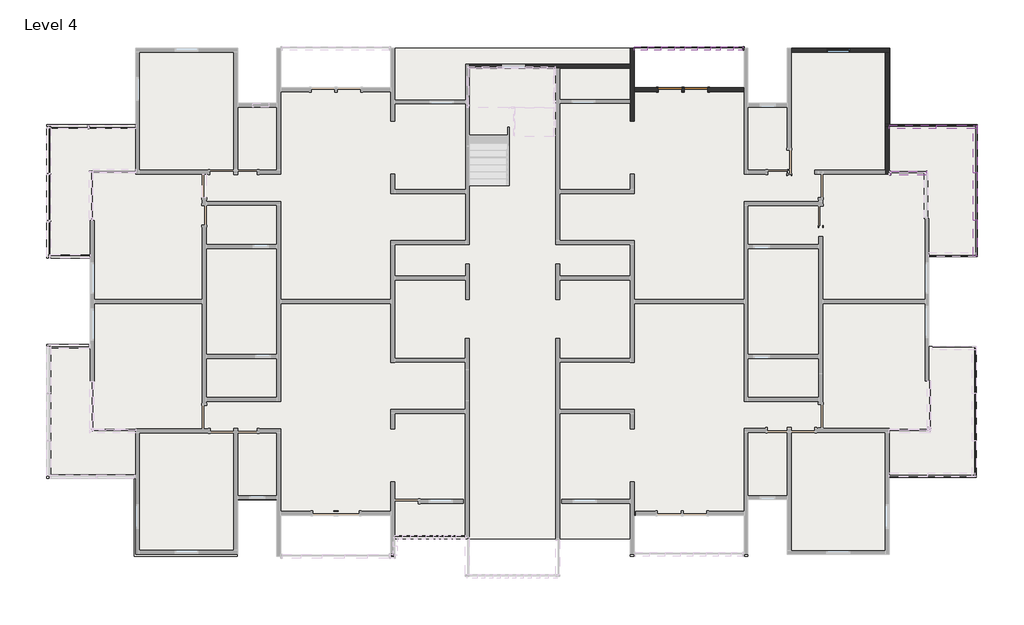
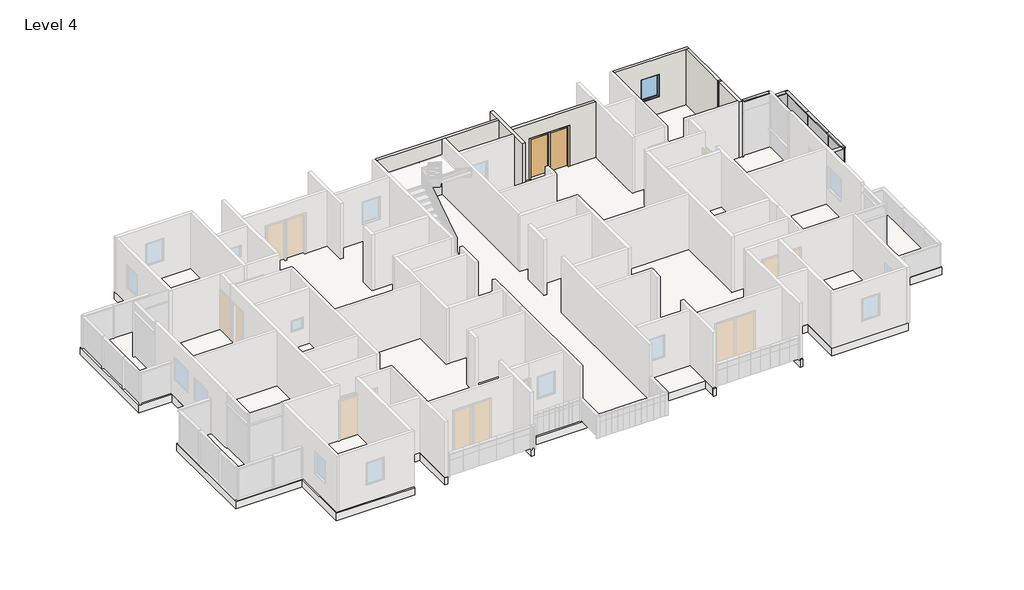
# One storey, part 5 of 7: 16 members, 15 plates, 7 walls, 2 doors, 1 slab, 1 window.
"""IFC4 building model written with IfcOpenShell, lengths in millimetres."""

import ifcopenshell
import ifcopenshell.guid

model = None  # the IFC model being written
_history = None  # IfcOwnerHistory: only IFC2X3 demands one
_inside = {}  # id of a spatial element -> (the spatial element, [elements in it])
_under = {}  # id of a project, library or spatial element -> (it, [spatial elements below it])
_declared = {}  # id of a project -> (the project, [libraries it declares])
_typed = {}  # id of a type object -> (the type object, [elements of that type])
_made_of = {}  # id of a material, layer set ... -> (it, [elements and type objects made of it])


def new_model(schema):
    """Start an empty IFC model of exactly this schema.

    Asked for "IFC4X3", IfcOpenShell would pick the latest addendum, in which some entities
    have other attributes; the version numbers below select the first issue.
    IFC2X3 requires an IfcOwnerHistory on every rooted entity: one is made here for all.
    """
    global model, _history
    if schema == "IFC4X3":
        model = ifcopenshell.file(schema_version=(4, 3, 0, 0))
    else:
        model = ifcopenshell.file(schema=schema)
    _inside.clear()
    _under.clear()
    _declared.clear()
    _typed.clear()
    _made_of.clear()
    _history = None
    if model.schema == "IFC2X3":
        org = make("IfcOrganization", Name="unknown")
        user = make(
            "IfcPersonAndOrganization",
            ThePerson=make("IfcPerson", FamilyName="unknown"),
            TheOrganization=org,
        )
        app = make(
            "IfcApplication",
            ApplicationDeveloper=org,
            Version="unknown",
            ApplicationFullName="unknown",
            ApplicationIdentifier="unknown",
        )
        _history = make(
            "IfcOwnerHistory",
            OwningUser=user,
            OwningApplication=app,
            ChangeAction="ADDED",
            CreationDate=0,
        )
    return model


def make(cls, **values):
    """One entity of the class cls with the attributes given. An attribute that is None is left unset."""
    return model.create_entity(
        cls, **{name: value for name, value in values.items() if value is not None}
    )


def rooted(cls, **values):
    """An entity with a GlobalId (a new one), such as an element, a storey or a relation."""
    return make(cls, GlobalId=ifcopenshell.guid.new(), OwnerHistory=_history, **values)


def si_unit(unit_type, name, prefix=None):
    """IfcSIUnit, for example si_unit("LENGTHUNIT", "METRE", prefix="MILLI")."""
    return make("IfcSIUnit", UnitType=unit_type, Prefix=prefix, Name=name)


def assignment(units):
    """IfcUnitAssignment: the units of a project."""
    return None if units is None else make("IfcUnitAssignment", Units=units)


def point(xyz):
    """IfcCartesianPoint."""
    return None if xyz is None else make("IfcCartesianPoint", Coordinates=xyz)


def direction(xyz):
    """IfcDirection."""
    return None if xyz is None else make("IfcDirection", DirectionRatios=xyz)


def frame(location, z_axis=None, x_axis=None):
    """IfcAxis2Placement3D, a coordinate frame: its origin and axes. An axis left out is left unset."""
    return make(
        "IfcAxis2Placement3D",
        Location=point(location),
        Axis=direction(z_axis),
        RefDirection=direction(x_axis),
    )


def origin():
    """The frame at (0, 0, 0) with its axes left unset."""
    return frame((0.0, 0.0, 0.0))


def origin_with_axes():
    """The frame at (0, 0, 0) with the z axis (0, 0, 1) and the x axis (1, 0, 0) written out."""
    return frame((0.0, 0.0, 0.0), z_axis=(0.0, 0.0, 1.0), x_axis=(1.0, 0.0, 0.0))


def place(relative_to, where):
    """IfcLocalPlacement: puts the frame where relative to a parent placement (None: the world)."""
    return make(
        "IfcLocalPlacement", PlacementRelTo=relative_to, RelativePlacement=where
    )


def context(
    kind, dimensions, precision=None, world=None, true_north=None, identifier=None
):
    """IfcGeometricRepresentationContext, for example the 3D "Model" context."""
    return make(
        "IfcGeometricRepresentationContext",
        ContextIdentifier=identifier,
        ContextType=kind,
        CoordinateSpaceDimension=dimensions,
        Precision=precision,
        WorldCoordinateSystem=world,
        TrueNorth=true_north,
    )


def project(units=None, contexts=None):
    """IfcProject with its units and contexts."""
    return rooted(
        "IfcProject",
        Name="project",
        RepresentationContexts=contexts,
        UnitsInContext=assignment(units),
    )


def spatial(cls, under=None, at=None, **own):
    """A site, building, storey or space (cls), placed at a placement, below another one or the project."""
    s = rooted(cls, ObjectPlacement=at, **own)
    if under is not None:
        _under.setdefault(under.id(), (under, []))[1].append(s)
    return s


def polyline(points):
    """IfcPolyline through the points."""
    return make("IfcPolyline", Points=[point(p) for p in points])


def outline(outer, holes=None, kind="AREA"):
    """IfcArbitraryClosedProfileDef: a profile drawn as a closed curve; with holes, ...WithVoids."""
    if holes is None:
        return make("IfcArbitraryClosedProfileDef", ProfileType=kind, OuterCurve=outer)
    return make(
        "IfcArbitraryProfileDefWithVoids",
        ProfileType=kind,
        OuterCurve=outer,
        InnerCurves=holes,
    )


def extrude(swept, where, along, depth):
    """IfcExtrudedAreaSolid: the profile swept, set in the frame where, extruded along a direction by depth."""
    return make(
        "IfcExtrudedAreaSolid",
        SweptArea=swept,
        Position=where,
        ExtrudedDirection=direction(along),
        Depth=depth,
    )


def faces_of(points, faces, orient=None, outer=None):
    """IfcFace entities. A face is a list of loops; a loop is a list of indices into points, from 0.

    orient and outer hold one flag for each loop. By default every Orientation is true, the
    first loop of a face is its IfcFaceOuterBound and the others are IfcFaceBound.
    """
    made = []
    for i, loops in enumerate(faces):
        bounds = []
        for j, loop in enumerate(loops):
            is_outer = j == 0 if outer is None else outer[i][j]
            bounds.append(
                make(
                    "IfcFaceOuterBound" if is_outer else "IfcFaceBound",
                    Bound=make("IfcPolyLoop", Polygon=[points[k] for k in loop]),
                    Orientation=True if orient is None else orient[i][j],
                )
            )
        made.append(make("IfcFace", Bounds=bounds))
    return made


def faceted_brep(points, faces, orient=None, outer=None, voids=None):
    """IfcFacetedBrep: a solid bounded by flat faces; with voids (closed shells), ...WithVoids."""
    shared = [point(p) for p in points]
    hull = make("IfcClosedShell", CfsFaces=faces_of(shared, faces, orient, outer))
    if voids is None:
        return make("IfcFacetedBrep", Outer=hull)
    return make(
        "IfcFacetedBrepWithVoids",
        Outer=hull,
        Voids=[
            make(cls, CfsFaces=faces_of(shared, fs, o, b)) for cls, fs, o, b in voids
        ],
    )


def shape(context_of_items, identifier, shape_type, items):
    """IfcShapeRepresentation: the items that make up one representation, for example the "Body"."""
    return make(
        "IfcShapeRepresentation",
        ContextOfItems=context_of_items,
        RepresentationIdentifier=identifier,
        RepresentationType=shape_type,
        Items=items,
    )


def source(mapping_origin, context_of_items, identifier, shape_type, items):
    """IfcRepresentationMap: a shape defined once, which mapped items show again and again."""
    return make(
        "IfcRepresentationMap",
        MappingOrigin=mapping_origin,
        MappedRepresentation=shape(context_of_items, identifier, shape_type, items),
    )


def transform(
    local_origin,
    x_axis=None,
    y_axis=None,
    z_axis=None,
    scale=None,
    scale2=None,
    scale3=None,
    uniform=True,
):
    """IfcCartesianTransformationOperator3D, or its non-uniform kind. x_axis, y_axis, z_axis: its Axis1, 2, 3."""
    if uniform:
        return make(
            "IfcCartesianTransformationOperator3D",
            Axis1=direction(x_axis),
            Axis2=direction(y_axis),
            LocalOrigin=point(local_origin),
            Scale=scale,
            Axis3=direction(z_axis),
        )
    return make(
        "IfcCartesianTransformationOperator3DnonUniform",
        Axis1=direction(x_axis),
        Axis2=direction(y_axis),
        LocalOrigin=point(local_origin),
        Scale=scale,
        Axis3=direction(z_axis),
        Scale2=scale2,
        Scale3=scale3,
    )


def mapped(mapping_source, mapping_target):
    """IfcMappedItem: shows the shape of a source again, moved by a transform."""
    return make(
        "IfcMappedItem", MappingSource=mapping_source, MappingTarget=mapping_target
    )


def made_of(thing, what):
    """Note that an element or type object is made of a material, layer set ...; save() writes the relation."""
    if what is not None:
        _made_of.setdefault(what.id(), (what, []))[1].append(thing)
    return thing


def element(
    cls,
    number,
    at=None,
    inside=None,
    cuts=None,
    type_object=None,
    material=None,
    context=None,
    identifier="Body",
    shape_type=None,
    held_by="IfcProductDefinitionShape",
    body=None,
    shapes=None,
    **own,
):
    """One element of the class cls, such as IfcWall. Its Tag is "e" and its number.

    at: its placement. inside: the storey or other place that contains it. cuts: it is an
    opening in that element (IfcRelVoidsElement). A single representation is given by context,
    identifier, shape_type and body (its items); several are given by shapes. held_by: the class
    of the entity that holds the representations. save() writes the other relations.
    """
    e = rooted(cls, Tag="e%d" % number, ObjectPlacement=at, **own)
    if body is not None:
        shapes = [shape(context, identifier, shape_type, body)]
    if shapes is not None:
        e.Representation = make(held_by, Representations=shapes)
    if inside is not None:
        _inside.setdefault(inside.id(), (inside, []))[1].append(e)
    if cuts is not None:
        rooted(
            "IfcRelVoidsElement", RelatingBuildingElement=cuts, RelatedOpeningElement=e
        )
    if type_object is not None:
        _typed.setdefault(type_object.id(), (type_object, []))[1].append(e)
    return made_of(e, material)


def aggregate(whole, parts):
    """IfcRelAggregates: a whole, such as a stair, and the parts it consists of."""
    return rooted("IfcRelAggregates", RelatingObject=whole, RelatedObjects=parts)


def save(model, path):
    """Write the relations noted so far, then the file.

    IfcRelAggregates (storeys below a building ...), IfcRelContainedInSpatialStructure (elements
    in a storey), IfcRelDefinesByType, IfcRelAssociatesMaterial and IfcRelDeclares: one each for
    every whole, place, type object, material and project.
    """
    for whole, parts in _under.values():
        aggregate(whole, parts)
    for where, things in _inside.values():
        rooted(
            "IfcRelContainedInSpatialStructure",
            RelatedElements=things,
            RelatingStructure=where,
        )
    for kind, things in _typed.values():
        rooted("IfcRelDefinesByType", RelatedObjects=things, RelatingType=kind)
    for what, things in _made_of.values():
        rooted("IfcRelAssociatesMaterial", RelatedObjects=things, RelatingMaterial=what)
    for by, libraries in _declared.values():
        rooted("IfcRelDeclares", RelatingContext=by, RelatedDefinitions=libraries)
    model.write(path)


def m_single_flush_0915_x_2134mm_138fd904(model_context):
    return source(origin(), model_context, "Body", "SweptSolid", [
        extrude(outline(polyline([(2210.0, -533.5), (0.0, -533.5), (0.0, -457.5), (2134.0, -457.5), (2134.0, 457.5), (0.0, 457.5), (0.0, 533.5), (2210.0, 533.5), (2210.0, -533.5)])), frame((0.0, 75.0, 0.0), z_axis=(0.0, 1.0, 0.0), x_axis=(0.0, 0.0, 1.0)), (0.0, 0.0, 1.0), 25.0),
        extrude(outline(polyline([(2210.0, 533.5), (2210.0, -533.5), (0.0, -533.5), (0.0, -457.5), (2134.0, -457.5), (2134.0, 457.5), (0.0, 457.5), (0.0, 533.5), (2210.0, 533.5)])), frame((0.0, -100.0, 0.0), z_axis=(0.0, 1.0, 0.0), x_axis=(0.0, 0.0, 1.0)), (0.0, 0.0, 1.0), 25.0),
        extrude(outline(polyline([(457.5, 24.0), (-457.5, 24.0), (-457.5, 75.0), (457.5, 75.0), (457.5, 24.0)])), origin_with_axes(), (0.0, 0.0, 1.0), 2134.0),
    ])


def rectangular_mullion_50mm_x_150mm_42770ee2(model_context):
    return source(origin(), model_context, "Body", "SweptSolid", [
        extrude(outline(polyline([(0.0, 75.0), (0.0, -75.0), (-50.0, -75.0), (-50.0, 75.0), (0.0, 75.0)])), frame((0.0, 0.0, -1830.0000003), z_axis=(0.0, 0.0, 1.0), x_axis=(1.0, 0.0, 0.0)), (0.0, 0.0, 1.0), 1830.0000003),
    ])


def rectangular_mullion_50mm_x_150mm_aaee7d48(model_context):
    return source(origin(), model_context, "Body", "SweptSolid", [
        extrude(outline(polyline([(0.0, 75.0), (0.0, -75.0), (-50.0, -75.0), (-50.0, 75.0), (0.0, 75.0)])), frame((0.0, 0.0, -1830.0), z_axis=(0.0, 0.0, 1.0), x_axis=(1.0, 0.0, 0.0)), (0.0, 0.0, 1.0), 1830.0),
    ])


def rectangular_mullion_50mm_x_150mm_efa02866(model_context):
    return source(origin(), model_context, "Body", "SweptSolid", [
        extrude(outline(polyline([(0.0, 75.0), (0.0, -75.0), (-50.0, -75.0), (-50.0, 75.0), (0.0, 75.0)])), frame((0.0, 0.0, -1399.9999997), z_axis=(0.0, 0.0, 1.0), x_axis=(1.0, 0.0, 0.0)), (0.0, 0.0, 1.0), 1399.9999997),
    ])


def rectangular_mullion_50mm_x_150mm_d9f1e9e9(model_context):
    return source(origin(), model_context, "Body", "SweptSolid", [
        extrude(outline(polyline([(0.0, 75.0), (0.0, -75.0), (-50.0, -75.0), (-50.0, 75.0), (0.0, 75.0)])), frame((0.0, 0.0, -1565.8160321), z_axis=(0.0, 0.0, 1.0), x_axis=(1.0, 0.0, 0.0)), (0.0, 0.0, 1.0), 1565.8160321),
    ])


def rectangular_mullion_50mm_x_150mm_89a65e42(model_context):
    return source(origin(), model_context, "Body", "SweptSolid", [
        extrude(outline(polyline([(0.0, 75.0), (0.0, -75.0), (-50.0, -75.0), (-50.0, 75.0), (0.0, 75.0)])), frame((0.0, 0.0, -1374.5), z_axis=(0.0, 0.0, 1.0), x_axis=(1.0, 0.0, 0.0)), (0.0, 0.0, 1.0), 1374.5),
    ])


def rectangular_mullion_50mm_x_150mm_729c0cfc(model_context):
    return source(origin(), model_context, "Body", "SweptSolid", [
        extrude(outline(polyline([(0.0, 75.0), (0.0, -75.0), (-50.0, -75.0), (-50.0, 75.0), (0.0, 75.0)])), frame((0.0, 0.0, -1250.0), z_axis=(0.0, 0.0, 1.0), x_axis=(1.0, 0.0, 0.0)), (0.0, 0.0, 1.0), 1250.0),
    ])


def rectangular_mullion_50mm_x_150mm_b3666dbd(model_context):
    return source(origin(), model_context, "Body", "SweptSolid", [
        extrude(outline(polyline([(0.0, 75.0), (0.0, -75.0), (-50.0, -75.0), (-50.0, 75.0), (0.0, 75.0)])), frame((0.0, 0.0, -500.0), z_axis=(0.0, 0.0, 1.0), x_axis=(1.0, 0.0, 0.0)), (0.0, 0.0, 1.0), 500.0),
    ])


def rectangular_mullion_50mm_x_150mm_e851a0b8(model_context):
    return source(origin(), model_context, "Body", "SweptSolid", [
        extrude(outline(polyline([(0.0, 75.0), (0.0, -75.0), (-50.0, -75.0), (-50.0, 75.0), (0.0, 75.0)])), frame((0.0, 0.0, -522.7272727), z_axis=(0.0, 0.0, 1.0), x_axis=(1.0, 0.0, 0.0)), (0.0, 0.0, 1.0), 522.7272727),
    ])


def rectangular_mullion_50mm_x_150mm_e11a3e7b(model_context):
    return source(origin(), model_context, "Body", "SweptSolid", [
        extrude(outline(polyline([(0.0, 75.0), (0.0, -75.0), (-50.0, -75.0), (-50.0, 75.0), (0.0, 75.0)])), frame((0.0, 0.0, -400.0), z_axis=(0.0, 0.0, 1.0), x_axis=(1.0, 0.0, 0.0)), (0.0, 0.0, 1.0), 400.0),
    ])


def rectangular_mullion_50mm_x_150mm_23485ade(model_context):
    return source(origin(), model_context, "Body", "SweptSolid", [
        extrude(outline(polyline([(0.0, 75.0), (0.0, -75.0), (-50.0, -75.0), (-50.0, 75.0), (0.0, 75.0)])), frame((0.0, 0.0, -350.0), z_axis=(0.0, 0.0, 1.0), x_axis=(1.0, 0.0, 0.0)), (0.0, 0.0, 1.0), 350.0),
    ])


def system_panel_glazed_09fbcc53(model_context):
    return source(origin(), model_context, "Body", "SweptSolid", [
        extrude(outline(polyline([(915.0000002, 24.5), (-915.0000002, 24.5), (-915.0000002, 49.5), (915.0000002, 49.5), (915.0000002, 24.5)])), origin_with_axes(), (0.0, 0.0, 1.0), 1200.0),
    ])


def system_panel_glazed_f4bbd109(model_context):
    return source(origin(), model_context, "Body", "SweptSolid", [
        extrude(outline(polyline([(910.8343113, 24.5), (-910.8343113, 24.5), (-910.8343113, 49.5), (910.8343113, 49.5), (910.8343113, 24.5)])), origin_with_axes(), (0.0, 0.0, 1.0), 1200.0),
    ])


def system_panel_glazed_42eec186(model_context):
    return source(origin(), model_context, "Body", "SweptSolid", [
        extrude(outline(polyline([(699.9999998, 24.5), (-699.9999998, 24.5), (-699.9999998, 49.5), (699.9999998, 49.5), (699.9999998, 24.5)])), origin_with_axes(), (0.0, 0.0, 1.0), 1200.0),
    ])


def system_panel_glazed_f2fc581d(model_context):
    return source(origin(), model_context, "Body", "SweptSolid", [
        extrude(outline(polyline([(782.9080161, 24.5), (-782.9080161, 24.5), (-782.9080161, 49.5), (782.9080161, 49.5), (782.9080161, 24.5)])), origin_with_axes(), (0.0, 0.0, 1.0), 1200.0),
    ])


def system_panel_glazed_346501af(model_context):
    return source(origin(), model_context, "Body", "SweptSolid", [
        extrude(outline(polyline([(250.0, 24.5), (-250.0, 24.5), (-250.0, 49.5), (250.0, 49.5), (250.0, 24.5)])), origin_with_axes(), (0.0, 0.0, 1.0), 1200.0),
    ])


def system_panel_glazed_5241e6d5(model_context):
    return source(origin(), model_context, "Body", "SweptSolid", [
        extrude(outline(polyline([(261.3636364, 24.5), (-261.3636364, 24.5), (-261.3636364, 49.5), (261.3636364, 49.5), (261.3636364, 24.5)])), origin_with_axes(), (0.0, 0.0, 1.0), 1200.0),
    ])


def system_panel_glazed_3e660766(model_context):
    return source(origin(), model_context, "Body", "SweptSolid", [
        extrude(outline(polyline([(200.0, 24.5), (-200.0, 24.5), (-200.0, 49.5), (200.0, 49.5), (200.0, 24.5)])), origin_with_axes(), (0.0, 0.0, 1.0), 1200.0),
    ])


def system_panel_glazed_b0a6d7cd(model_context):
    return source(origin(), model_context, "Body", "SweptSolid", [
        extrude(outline(polyline([(175.0, 24.5), (-175.0, 24.5), (-175.0, 49.5), (175.0, 49.5), (175.0, 24.5)])), origin_with_axes(), (0.0, 0.0, 1.0), 1200.0),
    ])


def m_fixed_0915_x_1220mm_873aa0e2(model_context):
    return source(origin(), model_context, "Body", "SweptSolid", [
        extrude(outline(polyline([(-394.5, 53.0), (394.5, 53.0), (394.5, 41.0), (-394.5, 41.0), (-394.5, 53.0)])), frame((0.0, 0.0, 978.0), z_axis=(0.0, 0.0, 1.0), x_axis=(1.0, 0.0, 0.0)), (0.0, 0.0, 1.0), 1094.0),
        extrude(outline(polyline([(2116.0, -438.5), (934.0, -438.5), (934.0, 438.5), (2116.0, 438.5), (2116.0, -438.5)]), holes=[polyline([(2072.0, -394.5), (2072.0, 394.5), (978.0, 394.5), (978.0, -394.5), (2072.0, -394.5)])]), frame((0.0, 25.0, 0.0), z_axis=(0.0, 1.0, 0.0), x_axis=(0.0, 0.0, 1.0)), (0.0, 0.0, 1.0), 44.0),
        extrude(outline(polyline([(2135.0, -457.5), (915.0, -457.5), (915.0, 457.5), (2135.0, 457.5), (2135.0, -457.5)]), holes=[polyline([(2116.0, -438.5), (2116.0, 438.5), (934.0, 438.5), (934.0, -438.5), (2116.0, -438.5)])]), frame((0.0, 25.0, 0.0), z_axis=(0.0, 1.0, 0.0), x_axis=(0.0, 0.0, 1.0)), (0.0, 0.0, 1.0), 63.0),
        extrude(outline(polyline([(2135.0, -457.5), (915.0, -457.5), (915.0, 457.5), (2135.0, 457.5), (2135.0, -457.5)]), holes=[polyline([(2103.0, -425.5), (2103.0, 425.5), (947.0, 425.5), (947.0, -425.5), (2103.0, -425.5)])]), frame((0.0, -62.0, 0.0), z_axis=(0.0, 1.0, 0.0), x_axis=(0.0, 0.0, 1.0)), (0.0, 0.0, 1.0), 87.0),
    ])


model = new_model("IFC4")

# Units and contexts
model_context = context("Model", 3, world=origin())
ifc_project = project(units=[si_unit("LENGTHUNIT", "METRE", prefix="MILLI")], contexts=[model_context])

# Site, building, storey
site = spatial("IfcSite", under=ifc_project)
building = spatial("IfcBuilding", under=site)
storey = spatial("IfcBuildingStorey", under=building, Name="Level 4", Elevation=9500.0)

# Doors
placement = place(None, origin())
m_single_flush_0915_x_2134mm_shape = m_single_flush_0915_x_2134mm_138fd904(model_context)
element("IfcDoor", 1, ObjectType="M_Single-Flush : 0915 x 2134mm", at=placement, inside=storey, context=model_context, shape_type="MappedRepresentation", body=[
    mapped(m_single_flush_0915_x_2134mm_shape, transform((6794.6515415, 8016.5690894, 9500.0), x_axis=(1.0, 0.0, 0.0), y_axis=(0.0, 1.0, 0.0), z_axis=(0.0, 0.0, 1.0))),
])
element("IfcDoor", 2, ObjectType="M_Single-Flush : 0915 x 2134mm", at=placement, inside=storey, context=model_context, shape_type="MappedRepresentation", body=[
    mapped(m_single_flush_0915_x_2134mm_shape, transform((5794.6515415, 8016.5690894, 9500.0), x_axis=(1.0, 0.0, 0.0), y_axis=(0.0, 1.0, 0.0), z_axis=(0.0, 0.0, 1.0))),
])

# Members
rectangular_mullion_50mm_x_150mm_shape = rectangular_mullion_50mm_x_150mm_42770ee2(model_context)
element("IfcMember", 3, ObjectType="Rectangular Mullion : 50mm x 150mm", at=placement, inside=storey, context=model_context, shape_type="MappedRepresentation", body=[
    mapped(rectangular_mullion_50mm_x_150mm_shape, transform((17635.0130284, 4788.3418163, 10750.0), x_axis=(0.0, 0.0, 1.0), y_axis=(-1.0, 0.0, 0.0), z_axis=(0.0, -1.0, 0.0))),
])
element("IfcMember", 4, ObjectType="Rectangular Mullion : 50mm x 150mm", at=placement, inside=storey, context=model_context, shape_type="MappedRepresentation", body=[
    mapped(rectangular_mullion_50mm_x_150mm_shape, transform((16129.1969963, 6568.8418166, 10750.0), x_axis=(0.0, 0.0, 1.0), y_axis=(0.0, -1.0, 0.0), z_axis=(1.0, 0.0, 0.0))),
])
rectangular_mullion_50mm_x_150mm_2_shape = rectangular_mullion_50mm_x_150mm_aaee7d48(model_context)
element("IfcMember", 5, ObjectType="Rectangular Mullion : 50mm x 150mm", at=placement, inside=storey, context=model_context, shape_type="MappedRepresentation", body=[
    mapped(rectangular_mullion_50mm_x_150mm_2_shape, transform((17635.0130284, 2958.3418163, 10750.0), x_axis=(0.0, 0.0, 1.0), y_axis=(-1.0, 0.0, 0.0), z_axis=(0.0, -1.0, 0.0))),
])
rectangular_mullion_50mm_x_150mm_3_shape = rectangular_mullion_50mm_x_150mm_efa02866(model_context)
element("IfcMember", 6, ObjectType="Rectangular Mullion : 50mm x 150mm", at=placement, inside=storey, context=model_context, shape_type="MappedRepresentation", body=[
    mapped(rectangular_mullion_50mm_x_150mm_3_shape, transform((17635.0130284, 1558.3418166, 10750.0), x_axis=(0.0, 0.0, 1.0), y_axis=(-1.0, 0.0, 0.0), z_axis=(0.0, -1.0, 0.0))),
])
rectangular_mullion_50mm_x_150mm_4_shape = rectangular_mullion_50mm_x_150mm_d9f1e9e9(model_context)
element("IfcMember", 7, ObjectType="Rectangular Mullion : 50mm x 150mm", at=placement, inside=storey, context=model_context, shape_type="MappedRepresentation", body=[
    mapped(rectangular_mullion_50mm_x_150mm_4_shape, transform((17695.0130284, 6568.8418166, 10750.0), x_axis=(0.0, 0.0, 1.0), y_axis=(0.0, -1.0, 0.0), z_axis=(1.0, 0.0, 0.0))),
])
rectangular_mullion_50mm_x_150mm_5_shape = rectangular_mullion_50mm_x_150mm_89a65e42(model_context)
element("IfcMember", 8, ObjectType="Rectangular Mullion : 50mm x 150mm", at=placement, inside=storey, context=model_context, shape_type="MappedRepresentation", body=[
    mapped(rectangular_mullion_50mm_x_150mm_5_shape, transform((15723.696996, 4778.8418166, 12500.0), x_axis=(0.0, 0.0, 1.0), y_axis=(0.0, -1.0, 0.0), z_axis=(1.0, 0.0, 0.0))),
])
rectangular_mullion_50mm_x_150mm_6_shape = rectangular_mullion_50mm_x_150mm_729c0cfc(model_context)
element("IfcMember", 9, ObjectType="Rectangular Mullion : 50mm x 150mm", at=placement, inside=storey, context=model_context, shape_type="MappedRepresentation", body=[
    mapped(rectangular_mullion_50mm_x_150mm_6_shape, transform((8667.3788142, 9614.2963621, 9500.0), x_axis=(1.0, 0.0, 0.0), y_axis=(0.0, -1.0, 0.0), z_axis=(0.0, 0.0, -1.0))),
])
rectangular_mullion_50mm_x_150mm_7_shape = rectangular_mullion_50mm_x_150mm_b3666dbd(model_context)
element("IfcMember", 10, ObjectType="Rectangular Mullion : 50mm x 150mm", at=placement, inside=storey, context=model_context, shape_type="MappedRepresentation", body=[
    mapped(rectangular_mullion_50mm_x_150mm_7_shape, transform((6867.3788142, 9614.2963621, 10750.0), x_axis=(0.0, 0.0, 1.0), y_axis=(0.0, -1.0, 0.0), z_axis=(1.0, 0.0, 0.0))),
])
element("IfcMember", 11, ObjectType="Rectangular Mullion : 50mm x 150mm", at=placement, inside=storey, context=model_context, shape_type="MappedRepresentation", body=[
    mapped(rectangular_mullion_50mm_x_150mm_7_shape, transform((7367.3788142, 9614.2963621, 10750.0), x_axis=(0.0, 0.0, 1.0), y_axis=(0.0, -1.0, 0.0), z_axis=(1.0, 0.0, 0.0))),
])
element("IfcMember", 12, ObjectType="Rectangular Mullion : 50mm x 150mm", at=placement, inside=storey, context=model_context, shape_type="MappedRepresentation", body=[
    mapped(rectangular_mullion_50mm_x_150mm_7_shape, transform((8267.3788142, 9614.2963621, 10750.0), x_axis=(0.0, 0.0, 1.0), y_axis=(0.0, -1.0, 0.0), z_axis=(1.0, 0.0, 0.0))),
])
rectangular_mullion_50mm_x_150mm_8_shape = rectangular_mullion_50mm_x_150mm_e851a0b8(model_context)
element("IfcMember", 13, ObjectType="Rectangular Mullion : 50mm x 150mm", at=placement, inside=storey, context=model_context, shape_type="MappedRepresentation", body=[
    mapped(rectangular_mullion_50mm_x_150mm_8_shape, transform((4921.9242687, 9614.2963621, 10750.0), x_axis=(0.0, 0.0, 1.0), y_axis=(0.0, -1.0, 0.0), z_axis=(1.0, 0.0, 0.0))),
])
element("IfcMember", 14, ObjectType="Rectangular Mullion : 50mm x 150mm", at=placement, inside=storey, context=model_context, shape_type="MappedRepresentation", body=[
    mapped(rectangular_mullion_50mm_x_150mm_8_shape, transform((5444.6515415, 9614.2963621, 10750.0), x_axis=(0.0, 0.0, 1.0), y_axis=(0.0, -1.0, 0.0), z_axis=(1.0, 0.0, 0.0))),
])
element("IfcMember", 15, ObjectType="Rectangular Mullion : 50mm x 150mm", at=placement, inside=storey, context=model_context, shape_type="MappedRepresentation", body=[
    mapped(rectangular_mullion_50mm_x_150mm_8_shape, transform((5967.3788142, 9614.2963621, 10750.0), x_axis=(0.0, 0.0, 1.0), y_axis=(0.0, -1.0, 0.0), z_axis=(1.0, 0.0, 0.0))),
])
rectangular_mullion_50mm_x_150mm_9_shape = rectangular_mullion_50mm_x_150mm_e11a3e7b(model_context)
element("IfcMember", 16, ObjectType="Rectangular Mullion : 50mm x 150mm", at=placement, inside=storey, context=model_context, shape_type="MappedRepresentation", body=[
    mapped(rectangular_mullion_50mm_x_150mm_9_shape, transform((6367.3788142, 9614.2963621, 10750.0), x_axis=(0.0, 0.0, 1.0), y_axis=(0.0, -1.0, 0.0), z_axis=(1.0, 0.0, 0.0))),
])
element("IfcMember", 17, ObjectType="Rectangular Mullion : 50mm x 150mm", at=placement, inside=storey, context=model_context, shape_type="MappedRepresentation", body=[
    mapped(rectangular_mullion_50mm_x_150mm_9_shape, transform((7767.3788142, 9614.2963621, 10750.0), x_axis=(0.0, 0.0, 1.0), y_axis=(0.0, -1.0, 0.0), z_axis=(1.0, 0.0, 0.0))),
])
rectangular_mullion_50mm_x_150mm_10_shape = rectangular_mullion_50mm_x_150mm_23485ade(model_context)
element("IfcMember", 18, ObjectType="Rectangular Mullion : 50mm x 150mm", at=placement, inside=storey, context=model_context, shape_type="MappedRepresentation", body=[
    mapped(rectangular_mullion_50mm_x_150mm_10_shape, transform((8617.3788142, 9614.2963621, 10750.0), x_axis=(0.0, 0.0, 1.0), y_axis=(0.0, -1.0, 0.0), z_axis=(1.0, 0.0, 0.0))),
])

# Plates
system_panel_glazed_shape = system_panel_glazed_09fbcc53(model_context)
element("IfcPlate", 19, ObjectType="System Panel : Glazed", at=placement, inside=storey, context=model_context, shape_type="MappedRepresentation", body=[
    mapped(system_panel_glazed_shape, transform((15214.1969962, 6568.8418166, 9500.0), x_axis=(1.0, 0.0, 0.0), y_axis=(0.0, 1.0, 0.0), z_axis=(0.0, 0.0, 1.0))),
])
element("IfcPlate", 20, ObjectType="System Panel : Glazed", at=placement, inside=storey, context=model_context, shape_type="MappedRepresentation", body=[
    mapped(system_panel_glazed_shape, transform((17635.0130284, 5703.3418165, 9500.0), x_axis=(0.0, -1.0, 0.0), y_axis=(1.0, 0.0, 0.0), z_axis=(0.0, 0.0, 1.0))),
])
element("IfcPlate", 21, ObjectType="System Panel : Glazed", at=placement, inside=storey, context=model_context, shape_type="MappedRepresentation", body=[
    mapped(system_panel_glazed_shape, transform((17635.0130284, 3873.3418163, 9500.0), x_axis=(0.0, -1.0, 0.0), y_axis=(1.0, 0.0, 0.0), z_axis=(0.0, 0.0, 1.0))),
])
system_panel_glazed_2_shape = system_panel_glazed_f4bbd109(model_context)
element("IfcPlate", 22, ObjectType="System Panel : Glazed", at=placement, inside=storey, context=model_context, shape_type="MappedRepresentation", body=[
    mapped(system_panel_glazed_2_shape, transform((16748.6787171, 1608.3418166, 9500.0), x_axis=(-1.0, 0.0, 0.0), y_axis=(0.0, -1.0, 0.0), z_axis=(0.0, 0.0, 1.0))),
])
system_panel_glazed_3_shape = system_panel_glazed_42eec186(model_context)
element("IfcPlate", 23, ObjectType="System Panel : Glazed", at=placement, inside=storey, context=model_context, shape_type="MappedRepresentation", body=[
    mapped(system_panel_glazed_3_shape, transform((17635.0130284, 2258.3418165, 9500.0), x_axis=(0.0, -1.0, 0.0), y_axis=(1.0, 0.0, 0.0), z_axis=(0.0, 0.0, 1.0))),
])
system_panel_glazed_4_shape = system_panel_glazed_f2fc581d(model_context)
element("IfcPlate", 24, ObjectType="System Panel : Glazed", at=placement, inside=storey, context=model_context, shape_type="MappedRepresentation", body=[
    mapped(system_panel_glazed_4_shape, transform((16912.1050124, 6568.8418166, 9500.0), x_axis=(1.0, 0.0, 0.0), y_axis=(0.0, 1.0, 0.0), z_axis=(0.0, 0.0, 1.0))),
])
system_panel_glazed_5_shape = system_panel_glazed_346501af(model_context)
element("IfcPlate", 25, ObjectType="System Panel : Glazed", at=placement, inside=storey, context=model_context, shape_type="MappedRepresentation", body=[
    mapped(system_panel_glazed_5_shape, transform((8017.3788142, 9614.2963621, 9500.0), x_axis=(1.0, 0.0, 0.0), y_axis=(0.0, 1.0, 0.0), z_axis=(0.0, 0.0, 1.0))),
])
element("IfcPlate", 26, ObjectType="System Panel : Glazed", at=placement, inside=storey, context=model_context, shape_type="MappedRepresentation", body=[
    mapped(system_panel_glazed_5_shape, transform((7117.3788142, 9614.2963621, 9500.0), x_axis=(1.0, 0.0, 0.0), y_axis=(0.0, 1.0, 0.0), z_axis=(0.0, 0.0, 1.0))),
])
element("IfcPlate", 27, ObjectType="System Panel : Glazed", at=placement, inside=storey, context=model_context, shape_type="MappedRepresentation", body=[
    mapped(system_panel_glazed_5_shape, transform((6617.3788142, 9614.2963621, 9500.0), x_axis=(1.0, 0.0, 0.0), y_axis=(0.0, 1.0, 0.0), z_axis=(0.0, 0.0, 1.0))),
])
system_panel_glazed_6_shape = system_panel_glazed_5241e6d5(model_context)
element("IfcPlate", 28, ObjectType="System Panel : Glazed", at=placement, inside=storey, context=model_context, shape_type="MappedRepresentation", body=[
    mapped(system_panel_glazed_6_shape, transform((4660.5606324, 9614.2963621, 9500.0), x_axis=(1.0, 0.0, 0.0), y_axis=(0.0, 1.0, 0.0), z_axis=(0.0, 0.0, 1.0))),
])
element("IfcPlate", 29, ObjectType="System Panel : Glazed", at=placement, inside=storey, context=model_context, shape_type="MappedRepresentation", body=[
    mapped(system_panel_glazed_6_shape, transform((5706.0151778, 9614.2963621, 9500.0), x_axis=(1.0, 0.0, 0.0), y_axis=(0.0, 1.0, 0.0), z_axis=(0.0, 0.0, 1.0))),
])
element("IfcPlate", 30, ObjectType="System Panel : Glazed", at=placement, inside=storey, context=model_context, shape_type="MappedRepresentation", body=[
    mapped(system_panel_glazed_6_shape, transform((5183.2879051, 9614.2963621, 9500.0), x_axis=(1.0, 0.0, 0.0), y_axis=(0.0, 1.0, 0.0), z_axis=(0.0, 0.0, 1.0))),
])
system_panel_glazed_7_shape = system_panel_glazed_3e660766(model_context)
element("IfcPlate", 31, ObjectType="System Panel : Glazed", at=placement, inside=storey, context=model_context, shape_type="MappedRepresentation", body=[
    mapped(system_panel_glazed_7_shape, transform((7567.3788142, 9614.2963621, 9500.0), x_axis=(1.0, 0.0, 0.0), y_axis=(0.0, 1.0, 0.0), z_axis=(0.0, 0.0, 1.0))),
])
element("IfcPlate", 32, ObjectType="System Panel : Glazed", at=placement, inside=storey, context=model_context, shape_type="MappedRepresentation", body=[
    mapped(system_panel_glazed_7_shape, transform((6167.3788142, 9614.2963621, 9500.0), x_axis=(1.0, 0.0, 0.0), y_axis=(0.0, 1.0, 0.0), z_axis=(0.0, 0.0, 1.0))),
])
system_panel_glazed_8_shape = system_panel_glazed_b0a6d7cd(model_context)
element("IfcPlate", 33, ObjectType="System Panel : Glazed", at=placement, inside=storey, context=model_context, shape_type="MappedRepresentation", body=[
    mapped(system_panel_glazed_8_shape, transform((8442.3788142, 9614.2963621, 9500.0), x_axis=(1.0, 0.0, 0.0), y_axis=(0.0, 1.0, 0.0), z_axis=(0.0, 0.0, 1.0))),
])

# Slab
element("IfcSlab", 34, ObjectType="Generic Floor - 400mm", at=placement, inside=storey, context=model_context, shape_type="SweptSolid", body=[
    extrude(outline(polyline([(-10978.0757313, 7482.4781803), (-9455.3484585, 7482.4781803), (-9455.3484585, 9614.2963621), (-9305.3484585, 9614.2963621), (-9305.3484585, 8091.5690894), (-5039.4393676, 8091.5690894), (-5039.4393676, 9614.2963621), (4399.196996, 9614.2963621), (4399.196996, 8091.5690894), (8665.1060869, 8091.5690894), (8665.1060869, 9614.2963621), (8817.3788142, 9614.2963621), (8817.3788142, 7482.4781803), (10342.3783683, 7482.4781803), (10342.3783683, 9614.2963621), (14312.8444058, 9614.2963621), (14312.8444058, 6653.3418166), (17717.8444058, 6653.3418166), (17717.8444058, 1533.3418166), (15837.8444058, 1533.3418166), (15837.8444058, -1946.1581834), (17677.8444058, -1946.1581834), (17677.8444058, -7028.8854561), (14240.1060869, -7028.8854561), (14240.1060869, -10028.8854561), (10340.1060869, -10028.8854561), (10340.1060869, -7894.794547), (8815.1060869, -7894.794547), (8815.1060869, -10106.1581834), (8665.1060869, -10106.1581834), (8665.1060869, -8506.1581834), (4401.4697233, -8506.1581834), (4401.4697233, -10106.1581834), (4251.4697233, -10106.1581834), (4251.4697233, -10028.8854561), (4251.4697233, -9417.5218198), (-4887.1666404, -9417.5218198), (-4887.1666404, -10006.7413208), (-4887.1666404, -10106.1581834), (-5039.4393676, -10106.1581834), (-5039.4393676, -8503.8854561), (-9303.0757313, -8503.8854561), (-9303.0757313, -10106.1581834), (-9453.0757313, -10106.1581834), (-9453.0757313, -7906.1581834), (-10989.3512663, -7906.1581834), (-10989.3512663, -10106.1581834), (-14989.3512663, -10106.1581834), (-14989.3512663, -7083.4309107), (-18389.3512663, -7083.4309107), (-18389.3512663, -1883.4309107), (-16697.1666404, -1883.4309107), (-16697.1666404, 1474.2963621), (-18377.1666404, 1474.2963621), (-18377.1666404, 6654.2963621), (-14937.1666404, 6654.2963621), (-14937.1666404, 9614.2963621), (-10978.0757313, 9614.2963621), (-10978.0757313, 7482.4781803)])), frame((0.0, 0.0, 9100.0), z_axis=(0.0, 0.0, 1.0), x_axis=(1.0, 0.0, 0.0)), (0.0, 0.0, 1.0), 400.0),
])

# Walls
element("IfcWall", 35, ObjectType="wal 150", at=placement, inside=storey, context=model_context, shape_type="Brep", body=[
    faceted_brep([(-1984.4393676, 8855.205453, 9500.0), (1358.2879051, 8855.205453, 9500.0), (1508.2879051, 8855.205453, 9500.0), (4249.196996, 8855.205453, 9500.0), (4249.196996, 8855.205453, 12500.0), (1508.2879051, 8855.205453, 12500.0), (1358.2879051, 8855.205453, 12500.0), (-1984.4393676, 8855.205453, 12500.0), (-733.0757313, 8855.205453, 10415.0), (-733.0757313, 8855.205453, 11635.0), (181.9242687, 8855.205453, 11635.0), (181.9242687, 8855.205453, 10415.0), (-1984.4393676, 9005.205453, 9500.0), (-1984.4393676, 9005.205453, 12500.0), (4249.196996, 9005.205453, 12500.0), (4249.196996, 9005.205453, 9500.0), (-733.0757313, 9005.205453, 10415.0), (181.9242687, 9005.205453, 10415.0), (181.9242687, 9005.205453, 11635.0), (-733.0757313, 9005.205453, 11635.0)], [[[0, 1, 2, 3, 4, 5, 6, 7], [8, 9, 10, 11]], [[12, 13, 14, 15], [16, 17, 18, 19]], [[3, 2, 1, 0, 12, 15]], [[7, 6, 5, 4, 14, 13]], [[4, 3, 15, 14]], [[9, 8, 16, 19]], [[10, 9, 19, 18]], [[11, 10, 18, 17]], [[8, 11, 17, 16]], [[0, 7, 13, 12]]]),
])
element("IfcWall", 36, ObjectType="wal 150", at=placement, inside=storey, context=model_context, shape_type="Brep", body=[
    faceted_brep([(4399.196996, 6792.1522268, 9500.0), (4399.196996, 7941.5690894, 9500.0), (4399.196996, 8091.5690894, 9500.0), (4399.196996, 9614.2963621, 9500.0), (4399.196996, 9614.2963621, 12500.0), (4399.196996, 8091.5690894, 12500.0), (4399.196996, 7941.5690894, 12500.0), (4399.196996, 6792.1522268, 12500.0), (4249.196996, 6792.1522268, 9500.0), (4249.196996, 6792.1522268, 12500.0), (4249.196996, 7484.7509075, 12500.0), (4249.196996, 7634.7509075, 12500.0), (4249.196996, 8855.205453, 12500.0), (4249.196996, 9005.205453, 12500.0), (4249.196996, 9614.2963621, 12500.0), (4249.196996, 9614.2963621, 9500.0), (4249.196996, 9005.205453, 9500.0), (4249.196996, 8855.205453, 9500.0), (4249.196996, 7634.7509075, 9500.0), (4249.196996, 7484.7509075, 9500.0)], [[[0, 1, 2, 3, 4, 5, 6, 7]], [[8, 9, 10, 11, 12, 13, 14, 15, 16, 17, 18, 19]], [[3, 2, 1, 0, 8, 19, 18, 17, 16, 15]], [[4, 3, 15, 14]], [[7, 6, 5, 4, 14, 13, 12, 11, 10, 9]], [[0, 7, 9, 8]]]),
])
element("IfcWall", 37, ObjectType="wal 150", at=placement, inside=storey, context=model_context, shape_type="SweptSolid", body=[
    extrude(outline(polyline([(9500.0, 8665.1060869), (12500.0, 8665.1060869), (12500.0, 4399.196996), (9500.0, 4399.196996), (9500.0, 5337.1515415), (11634.0, 5337.1515415), (11634.0, 6252.1515415), (9500.0, 6252.1515415), (9500.0, 6337.1515415), (11634.0, 6337.1515415), (11634.0, 7252.1515415), (9500.0, 7252.1515415), (9500.0, 8665.1060869)])), frame((0.0, 7941.5690894, 0.0), z_axis=(0.0, 1.0, 0.0), x_axis=(0.0, 0.0, 1.0)), (0.0, 0.0, 1.0), 150.0),
])
element("IfcWall", 38, ObjectType="wal 150", at=placement, inside=storey, context=model_context, shape_type="Brep", body=[
    faceted_brep([(10492.3783683, 9464.2963621, 9500.0), (14149.196996, 9464.2963621, 9500.0), (14299.196996, 9464.2963621, 9500.0), (14299.196996, 9464.2963621, 12500.0), (14149.196996, 9464.2963621, 12500.0), (10492.3783683, 9464.2963621, 12500.0), (11863.2876822, 9464.2963621, 10415.0), (11863.2876822, 9464.2963621, 11635.0), (12778.2876822, 9464.2963621, 11635.0), (12778.2876822, 9464.2963621, 10415.0), (10492.3783683, 9614.2963621, 9500.0), (10492.3783683, 9614.2963621, 12500.0), (14299.196996, 9614.2963621, 12500.0), (14299.196996, 9614.2963621, 9500.0), (11863.2876822, 9614.2963621, 10415.0), (12778.2876822, 9614.2963621, 10415.0), (12778.2876822, 9614.2963621, 11635.0), (11863.2876822, 9614.2963621, 11635.0)], [[[0, 1, 2, 3, 4, 5], [6, 7, 8, 9]], [[10, 11, 12, 13], [14, 15, 16, 17]], [[2, 1, 0, 10, 13]], [[5, 4, 3, 12, 11]], [[7, 6, 14, 17]], [[8, 7, 17, 16]], [[9, 8, 16, 15]], [[6, 9, 15, 14]], [[0, 5, 11, 10]], [[3, 2, 13, 12]]]),
])
element("IfcWall", 39, ObjectType="wal 150", at=placement, inside=storey, context=model_context, shape_type="SweptSolid", body=[
    extrude(outline(polyline([(14149.196996, 6668.8418166), (14149.196996, 9464.2963621), (14299.196996, 9464.2963621), (14299.196996, 6668.8418166), (14149.196996, 6668.8418166)])), frame((0.0, 0.0, 9500.0), z_axis=(0.0, 0.0, 1.0), x_axis=(1.0, 0.0, 0.0)), (0.0, 0.0, 1.0), 3000.0),
])
element("IfcWall", 40, ObjectType="wal 150", at=placement, inside=storey, context=model_context, shape_type="Brep", body=[
    faceted_brep([(14149.196996, 6568.8418166, 9500.0), (14149.196996, 4893.8418166, 9500.0), (14149.196996, 4743.8418166, 9500.0), (14149.196996, 4741.5690894, 9500.0), (14149.196996, 4741.5690894, 12500.0), (14149.196996, 4743.8418166, 12500.0), (14149.196996, 4893.8418166, 12500.0), (14149.196996, 6568.8418166, 12500.0), (14299.196996, 6568.8418166, 9500.0), (14299.196996, 6568.8418166, 12500.0), (14299.196996, 4741.5690894, 12500.0), (14299.196996, 4741.5690894, 9500.0)], [[[0, 1, 2, 3, 4, 5, 6, 7]], [[8, 9, 10, 11]], [[3, 2, 1, 0, 8, 11]], [[4, 3, 11, 10]], [[7, 6, 5, 4, 10, 9]], [[0, 7, 9, 8]]]),
])
element("IfcWall", 41, ObjectType="wal 150", at=placement, inside=storey, context=model_context, shape_type="SweptSolid", body=[
    extrude(outline(polyline([(14149.196996, 6568.8418166), (14149.196996, 6668.8418166), (14299.196996, 6668.8418166), (14299.196996, 6568.8418166), (14149.196996, 6568.8418166)])), frame((0.0, 0.0, 9500.0), z_axis=(0.0, 0.0, 1.0), x_axis=(1.0, 0.0, 0.0)), (0.0, 0.0, 1.0), 3000.0),
])

# Window
m_fixed_0915_x_1220mm_shape = m_fixed_0915_x_1220mm_873aa0e2(model_context)
element("IfcWindow", 42, ObjectType="M_Fixed : 1.80 to 1.20 w2", at=placement, inside=storey, context=model_context, shape_type="MappedRepresentation", body=[
    mapped(m_fixed_0915_x_1220mm_shape, transform((12320.7876822, 9526.2963621, 9500.0), x_axis=(1.0, 0.0, 0.0), y_axis=(0.0, 1.0, 0.0), z_axis=(0.0, 0.0, 1.0))),
])

save(model, "model.ifc")

# Revit data of these elements
# Type "M_Single-Flush : 0915 x 2134mm"
#   Type Mark = "15"
#   Thickness = 0.051 m
#   Height = 2.134 m
#   Trim Projection Ext = 0.025 m
#   Trim Projection Int = 0.025 m
#   Trim Width = 0.076 m
#   Width = 0.915 m
#   Door Material = Door - Panel
#   Frame Material = Door - Frame
#   Function = (empty or 0)
#   Wall Closure = (empty or 0)
# Type "Rectangular Mullion : 50mm x 150mm"
#   built-in parameter 1007304 = 0.492126 (stored number, unit not read)
#   built-in parameter 1007301 = 0.082021 (stored number, unit not read)
#   built-in parameter 1007300 = 0.082021 (stored number, unit not read)
# Type "Generic Floor - 400mm"
#   Function = 0
#   Layers, outside or top first: 0.4 m no material (function 1)
# Type "wal 150"
#   Layers, outside or top first: 0.15 m no material (function 1)
# Type "M_Fixed : 1.80 to 1.20 w2"
#   Type Mark = "19"
#   Height = 1.22 m
#   Default Sill Height = 0.915 m
#   Width = 0.915 m
#   Window Inset = 0.019 m
#   Frame Exterior Material = Sash
#   Frame Interior Material = Sash
#   Glass Pane Material = Glass
#   Sash = Sash
#   Wall Closure = (empty or 0)
# Elements 1, 2 (IfcDoor, "M_Single-Flush : 0915 x 2134mm")
#   Phase Created = New Construction
#   Materials on its faces: "Door - Frame", "Door - Panel"
# Elements 3, 4, 5, 6, 7, 8, 9, 10, 11, 12, 13, 14, 15, 16, 17, 18 (IfcMember, "Rectangular Mullion : 50mm x 150mm")
#   Phase Created = New Construction
#   Materials on its faces: "Aluminum"
# Elements 19, 20, 21, 22, 23, 24, 25, 26, 27, 28, 29, 30, 31, 32, 33 (IfcPlate, "System Panel : Glazed")
#   Phase Created = New Construction
#   Materials on its faces: "Glass"
# Element 34 (IfcSlab, "Generic Floor - 400mm")
#   built-in parameter 1001955 = 3.14159 (stored number, unit not read)
#   Height Offset From Level = 0 m
#   Phase Created = New Construction
#   Materials on its faces: "Default Roof", "Door - Frame", "Ceiling Tile 600 x 1200", "Oak Flooring"
# Elements 35, 39, 40 (IfcWall, "wal 150")
#   Top Offset = 0 m
#   Base Offset = 0 m
#   Unconnected Height = 3 m
#   wall height = 3 m
#   Phase Created = New Construction
#   Base Constraint = Level 4
#   Materials on its faces: "Default Wall", "Ceiling Tile 600 x 1200"
# Element 36 (IfcWall, "wal 150")
#   Top Offset = 0 m
#   Base Offset = 0 m
#   Unconnected Height = 3 m
#   wall height = 3 m
#   Phase Created = New Construction
#   Base Constraint = Level 4
#   Materials on its faces: "Default Wall", "Ceiling Tile 600 x 600"
# Element 37 (IfcWall, "wal 150")
#   Top Offset = 0 m
#   Base Offset = 0 m
#   Unconnected Height = 3 m
#   wall height = 3 m
#   Phase Created = New Construction
#   Base Constraint = Level 4
#   Materials on its faces: "Default Wall", "Door - Frame"
# Element 38 (IfcWall, "wal 150")
#   Top Offset = 0 m
#   Base Offset = 0 m
#   Unconnected Height = 3 m
#   wall height = 3 m
#   Phase Created = New Construction
#   Base Constraint = Level 4
#   Materials on its faces: "Default Wall", "Ceiling Tile 600 x 600", "Ceiling Tile 600 x 1200"
# Element 41 (IfcWall, "wal 150")
#   Top Offset = 0 m
#   Base Offset = 0 m
#   Unconnected Height = 3 m
#   wall height = 3 m
#   Phase Created = New Construction
#   Base Constraint = Level 4
#   Materials on its faces: "Default Wall", "Brick, Common"
# Element 42 (IfcWindow, "M_Fixed : 1.80 to 1.20 w2")
#   Mark = "327"
#   Phase Created = New Construction
#   Materials on its faces: "Sash", "Glass"
# Materials
#   "Door - Panel": class "Wood", colour RGB 114 82 51, transparency 0
#   "Door - Frame": class "Miscellaneous", colour RGB 255 0 128, transparency 0, Cost = 0
#   "Sash": class "Wood", colour RGB 136 99 55, transparency 0
#   "Glass": class "Glass", colour RGB 218 227 224, transparency 0.85, Description = "Soda Lime Glass", Cost = 0
#   "Aluminum": class "Metal", colour RGB 244 244 244, transparency 0, Description = "Aluminum 6061", Cost = 0
#   "Default Roof": class "Miscellaneous", colour RGB 80 80 80, transparency 0
#   "Ceiling Tile 600 x 1200": class "Generic", colour RGB 179 178 175, transparency 0, Description = "Acoustic ceiling tile", Cost = 0
#   "Oak Flooring": class "Wood", colour RGB 216 169 114, transparency 0, Description = "Quercus Rubra", Cost = 0
#   "Default Wall": class "Miscellaneous", colour RGB 80 80 80, transparency 0
#   "Ceiling Tile 600 x 600": class "Generic", colour RGB 180 179 177, transparency 0, Description = "Acoustic ceiling tile", Cost = 0
#   "Brick, Common": class "Masonry", colour RGB 76 55 59, transparency 0, Description = "Common brick", Cost = 0
